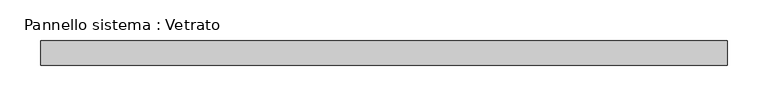
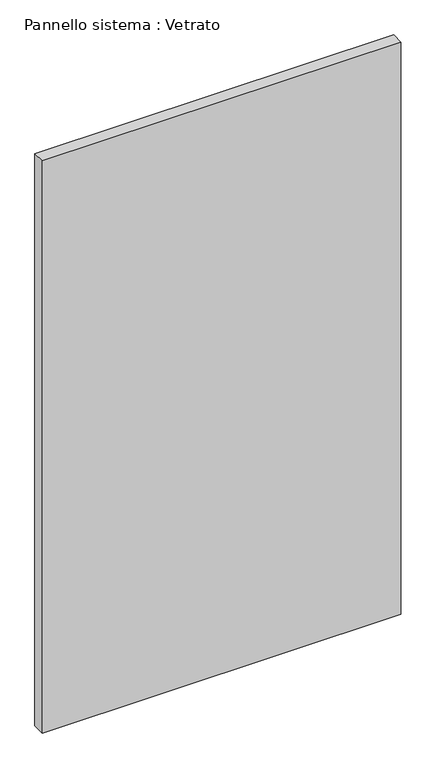
"""IFC4 building model written with IfcOpenShell, lengths in millimetres: plate geometry, Pannello sistema : Vetrato."""

from ifc_helpers import new_model, si_unit, origin, origin_with_axes, place, context, project, spatial, polyline, outline, extrude, source, transform, mapped, element, save


def pannello_sistema_vetrato_0d3d6609(model_context):
    return source(origin(), model_context, "Body", "SweptSolid", [
        extrude(outline(polyline([(422.5, -15.0), (-422.5, -15.0), (-422.5, 15.0), (422.5, 15.0), (422.5, -15.0)])), origin_with_axes(), (0.0, 0.0, 1.0), 1425.0),
    ])


if __name__ == "__main__":
    model = new_model("IFC4")
    model_context = context("Model", 3, world=origin())
    ifc_project = project(units=[si_unit("LENGTHUNIT", "METRE", prefix="MILLI")], contexts=[model_context])
    site = spatial("IfcSite", under=ifc_project)
    building = spatial("IfcBuilding", under=site)
    placement = place(None, origin())
    pannello_sistema_vetrato_shape = pannello_sistema_vetrato_0d3d6609(model_context)
    element("IfcPlate", 1, ObjectType="Pannello sistema : Vetrato", at=placement, inside=building, context=model_context, shape_type="MappedRepresentation", body=[
        mapped(pannello_sistema_vetrato_shape, transform((0.0, 0.0, 0.0), x_axis=(1.0, 0.0, 0.0), y_axis=(0.0, 1.0, 0.0), z_axis=(0.0, 0.0, 1.0))),
    ])
    save(model, "model.ifc")

# Revit data of these elements
# Type "Pannello sistema : Vetrato"
#   Construction Type Id = "GSP4R"
#   Analytic Construction = "Vetrata singola Pilkington 1/8 in"
#   Visual Light Transmittance = 0.9
#   Solar Heat Gain Coefficient = 0.86
#   Heat Transfer Coefficient (U) = 6.7069 W/(m²·K)
# Element 1 (IfcPlate, "Pannello sistema : Vetrato")
#   Materials on its faces: "Default - Vetro"
# Materials
#   "Default - Vetro": class "Vetro", colour RGB 208 208 208, transparency 0.7, Cost = 0
